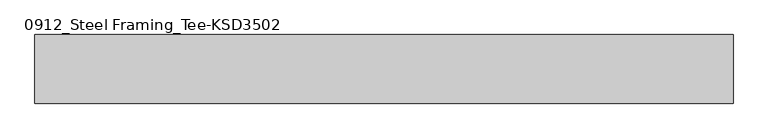
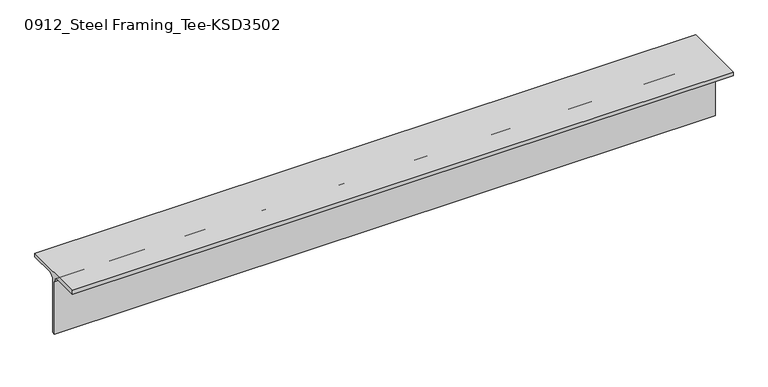
"""IFC4 building model written with IfcOpenShell, lengths in millimetres: member geometry, 0912_Steel Framing_Tee-KSD3502 : H_SB_ASB_CT-150x150x6.5x9."""

from ifc_helpers import new_model, si_unit, point, frame, frame_2d, origin, place, context, project, spatial, polyline, circle_curve, trimmed, segment, composite_curve, outline, extrude, source, transform, mapped, element, save


def member_0912_steel_framing_tee_ksd3502_1ea47a5b(model_context):
    return source(origin(), model_context, "Body", "SweptSolid", [
        extrude(outline(composite_curve([segment(polyline([(75.0, 75.0), (75.0, 66.0), (16.25, 66.0)]), True, "CONTINUOUS"), segment(trimmed(circle_curve(frame_2d((16.25, 53.0)), 13.0), [point((16.25, 66.0))], [point((3.25, 53.0))], True, "CARTESIAN"), True, "CONTINUOUS"), segment(polyline([(3.25, 53.0), (3.25, -75.0), (-3.25, -75.0), (-3.25, 53.0)]), True, "CONTINUOUS"), segment(trimmed(circle_curve(frame_2d((-16.25, 53.0)), 13.0), [point((-3.25, 53.0))], [point((-16.25, 66.0))], True, "CARTESIAN"), True, "CONTINUOUS"), segment(polyline([(-16.25, 66.0), (-75.0, 66.0), (-75.0, 75.0), (75.0, 75.0)]), True, "CONTINUOUS")], self_intersect=False)), frame((-719.0, 0.0, 0.0), z_axis=(1.0, 0.0, 0.0), x_axis=(0.0, 1.0, 0.0)), (0.0, 0.0, 1.0), 1526.1),
    ])


if __name__ == "__main__":
    model = new_model("IFC4")
    model_context = context("Model", 3, world=origin())
    ifc_project = project(units=[si_unit("LENGTHUNIT", "METRE", prefix="MILLI")], contexts=[model_context])
    site = spatial("IfcSite", under=ifc_project)
    building = spatial("IfcBuilding", under=site)
    placement = place(None, origin())
    member_0912_steel_framing_tee_ksd3502_shape = member_0912_steel_framing_tee_ksd3502_1ea47a5b(model_context)
    element("IfcMember", 1, ObjectType="0912_Steel Framing_Tee-KSD3502 : H_SB_ASB_CT-150x150x6.5x9", at=placement, inside=building, context=model_context, shape_type="MappedRepresentation", body=[
        mapped(member_0912_steel_framing_tee_ksd3502_shape, transform((0.0, 0.0, 0.0), x_axis=(1.0, 0.0, 0.0), y_axis=(0.0, 1.0, 0.0), z_axis=(0.0, 0.0, 1.0))),
    ])
    save(model, "model.ifc")

# Revit data of these elements
# Type "0912_Steel Framing_Tee-KSD3502 : H_SB_ASB_CT-150x150x6.5x9"
#   H_WM Code_1 = "S01AA003-00001 | Main Steel Structure Fabrication Work | Shelter/Building | Light Steel - Standard (30KG/M>Weight) | Material: (   )"
#   H_WM Code_2 = "S03AA029-00001 | Main Steel Structure Erection Work | Shelter/Building | Light Steel (30KG/M>Weight) | Material: (   )"
#   H_WM Code_3 = "S01AA010-00001 | Main Steel Structure Fabrication Work | Shelter/Building | Steel Painting/Coating | for Non-Fireproofed Steel Surface, Surface Preparation, Primer, Second & Final Coat | Material: (   )"
#   H_Q'ty Cal Type Tag = "SB-Q2"
#   Width = 15.0 cm
#   Web Thickness = 0.65 cm
#   Web Fillet = 1.3 cm
#   Section Area = 23.39 cm²
#   Perimeter = 0.60 m²/m
#   Nominal Weight = 18.40 kgf/m
#   Height = 15.0 cm
#   Flange Thickness = 0.9 cm
#   Centroid Vertical = 7.5 cm
#   Centroid Horizontal = 7.5 cm
#   Length [instance default] = 1.5000 m
#   Structural Material [instance default] = Steel, 45-345
#   Warping Constant = (empty or 0)
#   Torsional Moment of Inertia = 0
#   Section Name Key = ""
#   Plastic Modulus weak axis = 0
#   Plastic Modulus strong axis = 0
#   Moment of Inertia weak axis = 0
#   Moment of Inertia strong axis = 0
#   Elastic Modulus weak axis = 0
#   Elastic Modulus strong axis = 0
#   Bolt Spacing = 0
#   Assembly Code = ""
# Element 1 (IfcMember, "0912_Steel Framing_Tee-KSD3502 : H_SB_ASB_CT-150x150x6.5x9")
#   Structural Material = none
# Materials
#   "Steel, 45-345": class "Metal", colour RGB 189 187 185, transparency 0, Description = "Steel 345 MPa", Cost = 0
